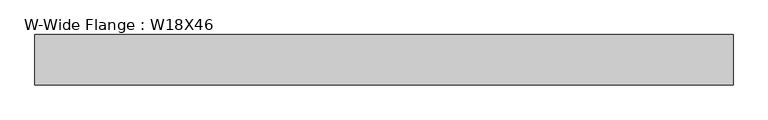
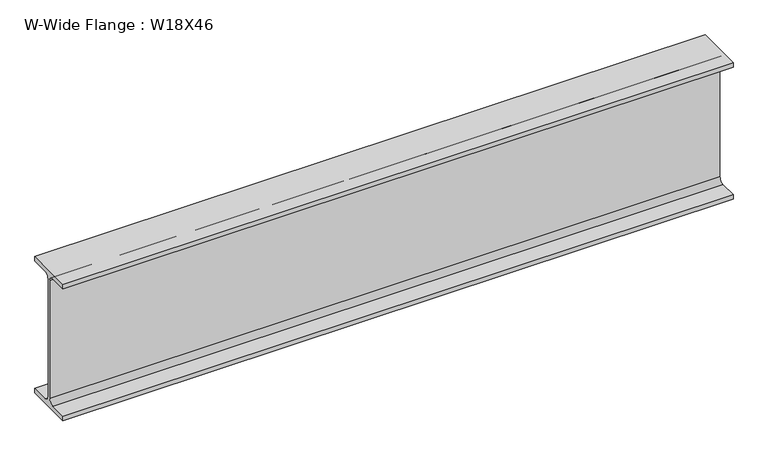
"""IFC4 building model written with IfcOpenShell, lengths in millimetres: beam geometry, W-Wide Flange : W18X46."""

from ifc_helpers import new_model, si_unit, point, frame, frame_2d, origin, place, context, project, spatial, polyline, circle_curve, trimmed, segment, composite_curve, outline, extrude, source, transform, mapped, element, save


def w_wide_flange_w18x46_89d715c2(model_context):
    return source(origin(), model_context, "Body", "SweptSolid", [
        extrude(outline(composite_curve([segment(polyline([(76.962, -214.503), (76.962, -229.87), (-76.962, -229.87), (-76.962, -214.503), (-20.955, -214.503)]), True, "CONTINUOUS"), segment(trimmed(circle_curve(frame_2d((-20.955, -198.12)), 16.383), [point((-20.955, -214.503))], [point((-4.572, -198.12))], True, "CARTESIAN"), True, "CONTINUOUS"), segment(polyline([(-4.572, -198.12), (-4.572, 198.12)]), True, "CONTINUOUS"), segment(trimmed(circle_curve(frame_2d((-20.955, 198.12)), 16.383), [point((-4.572, 198.12))], [point((-20.955, 214.503))], True, "CARTESIAN"), True, "CONTINUOUS"), segment(polyline([(-20.955, 214.503), (-76.962, 214.503), (-76.962, 229.87), (76.962, 229.87), (76.962, 214.503), (20.955, 214.503)]), True, "CONTINUOUS"), segment(trimmed(circle_curve(frame_2d((20.955, 198.12)), 16.383), [point((20.955, 214.503))], [point((4.572, 198.12))], True, "CARTESIAN"), True, "CONTINUOUS"), segment(polyline([(4.572, 198.12), (4.572, -198.12)]), True, "CONTINUOUS"), segment(trimmed(circle_curve(frame_2d((20.955, -198.12)), 16.383), [point((4.572, -198.12))], [point((20.955, -214.503))], True, "CARTESIAN"), True, "CONTINUOUS"), segment(polyline([(20.955, -214.503), (76.962, -214.503)]), True, "CONTINUOUS")], self_intersect=False)), frame((-1054.1, 0.0, 0.0), z_axis=(1.0, 0.0, 0.0), x_axis=(0.0, 1.0, 0.0)), (0.0, 0.0, 1.0), 2133.6),
    ])


if __name__ == "__main__":
    model = new_model("IFC4")
    model_context = context("Model", 3, world=origin())
    ifc_project = project(units=[si_unit("LENGTHUNIT", "METRE", prefix="MILLI")], contexts=[model_context])
    site = spatial("IfcSite", under=ifc_project)
    building = spatial("IfcBuilding", under=site)
    placement = place(None, origin())
    w_wide_flange_w18x46_shape = w_wide_flange_w18x46_89d715c2(model_context)
    element("IfcBeam", 1, ObjectType="W-Wide Flange : W18X46", at=placement, inside=building, context=model_context, shape_type="MappedRepresentation", body=[
        mapped(w_wide_flange_w18x46_shape, transform((0.0, 0.0, 0.0), x_axis=(1.0, 0.0, 0.0), y_axis=(0.0, 1.0, 0.0), z_axis=(0.0, 0.0, 1.0))),
    ])
    save(model, "model.ifc")

# Revit data of these elements
# Type "W-Wide Flange : W18X46"
#   Assembly Code = "B10"
#   W = 46
#   Length [instance default] = 5' - 0"
#   bf = 0' - 6.06"
#   d = 1' - 6.1"
#   k = 0' - 1 1/4"
#   k2 = 0' - 0.645"
#   tf = 0' - 0.605"
#   tw = 0' - 0.36"
#   A = 0.09375 SF
#   Structural Material [instance default] = Steel ASTM A992
# Element 1 (IfcBeam, "W-Wide Flange : W18X46")
#   Materials on its faces: "Steel ASTM A992"
# Materials
#   "Steel ASTM A992": class "Metal", colour RGB 199 199 199, transparency 0, Description = "Structural steel 50ksi", Cost = 0
